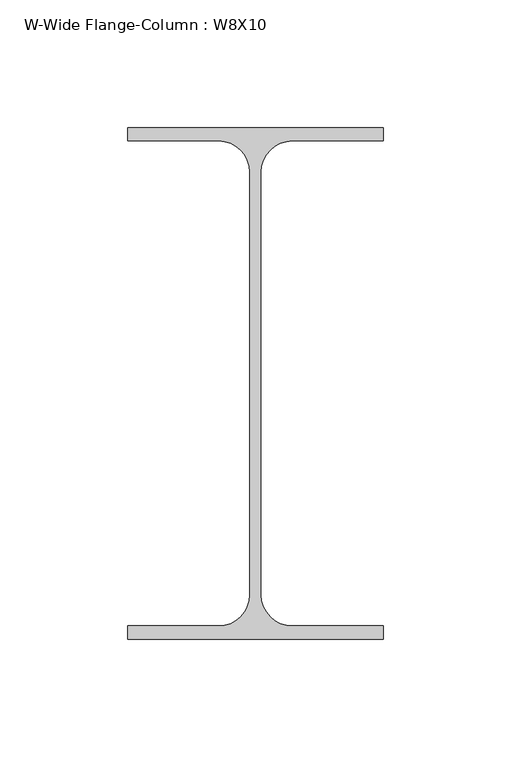
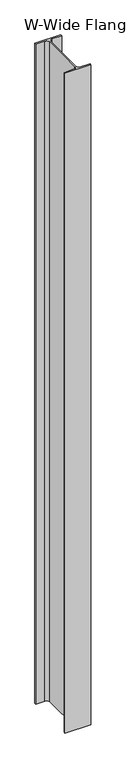
"""IFC4 building model written with IfcOpenShell, lengths in millimetres: column geometry, W-Wide Flange-Column : W8X10."""

from ifc_helpers import new_model, si_unit, point, frame_2d, origin, origin_with_axes, place, context, project, spatial, polyline, circle_curve, trimmed, segment, composite_curve, outline, extrude, source, transform, mapped, element, save


def w_wide_flange_column_w8x10_bb29b329(model_context):
    return source(origin(), model_context, "Body", "SweptSolid", [
        extrude(outline(composite_curve([segment(polyline([(50.038, 100.203), (50.038, 94.996), (14.4145, 94.996)]), True, "CONTINUOUS"), segment(trimmed(circle_curve(frame_2d((14.4145, 82.7405)), 12.2555), [point((14.4145, 94.996))], [point((2.159, 82.7405))], True, "CARTESIAN"), True, "CONTINUOUS"), segment(polyline([(2.159, 82.7405), (2.159, -82.7405)]), True, "CONTINUOUS"), segment(trimmed(circle_curve(frame_2d((14.4145, -82.7405)), 12.2555), [point((2.159, -82.7405))], [point((14.4145, -94.996))], True, "CARTESIAN"), True, "CONTINUOUS"), segment(polyline([(14.4145, -94.996), (50.038, -94.996), (50.038, -100.203), (-50.038, -100.203), (-50.038, -94.996), (-14.4145, -94.996)]), True, "CONTINUOUS"), segment(trimmed(circle_curve(frame_2d((-14.4145, -82.7405)), 12.2555), [point((-14.4145, -94.996))], [point((-2.159, -82.7405))], True, "CARTESIAN"), True, "CONTINUOUS"), segment(polyline([(-2.159, -82.7405), (-2.159, 82.7405)]), True, "CONTINUOUS"), segment(trimmed(circle_curve(frame_2d((-14.4145, 82.7405)), 12.2555), [point((-2.159, 82.7405))], [point((-14.4145, 94.996))], True, "CARTESIAN"), True, "CONTINUOUS"), segment(polyline([(-14.4145, 94.996), (-50.038, 94.996), (-50.038, 100.203), (50.038, 100.203)]), True, "CONTINUOUS")], self_intersect=False)), origin_with_axes(), (0.0, 0.0, 1.0), 2692.4),
    ])


if __name__ == "__main__":
    model = new_model("IFC4")
    model_context = context("Model", 3, world=origin())
    ifc_project = project(units=[si_unit("LENGTHUNIT", "METRE", prefix="MILLI")], contexts=[model_context])
    site = spatial("IfcSite", under=ifc_project)
    building = spatial("IfcBuilding", under=site)
    placement = place(None, origin())
    w_wide_flange_column_w8x10_shape = w_wide_flange_column_w8x10_bb29b329(model_context)
    element("IfcColumn", 1, ObjectType="W-Wide Flange-Column : W8X10", at=placement, inside=building, context=model_context, shape_type="MappedRepresentation", body=[
        mapped(w_wide_flange_column_w8x10_shape, transform((0.0, 0.0, 0.0), x_axis=(1.0, 0.0, 0.0), y_axis=(0.0, 1.0, 0.0), z_axis=(0.0, 0.0, 1.0))),
    ])
    save(model, "model.ifc")

# Revit data of these elements
# Type "W-Wide Flange-Column : W8X10"
#   Assembly Code = "B10"
#   W = 10
#   bf = 0' - 3.94"
#   d = 0' - 7.89"
#   k = 0' - 0 11/16"
#   kr = 0' - 0.4825"
#   tf = 0' - 0.205"
#   tw = 0' - 0.17"
#   A = 0.0205556 SF
#   Structural Material [instance default] = Steel ASTM A992
# Element 1 (IfcColumn, "W-Wide Flange-Column : W8X10")
#   Materials on its faces: "Steel ASTM A992"
# Materials
#   "Steel ASTM A992": class "Metal", colour RGB 189 187 185, transparency 0, Description = "Structural steel 50ksi", Cost = 0
